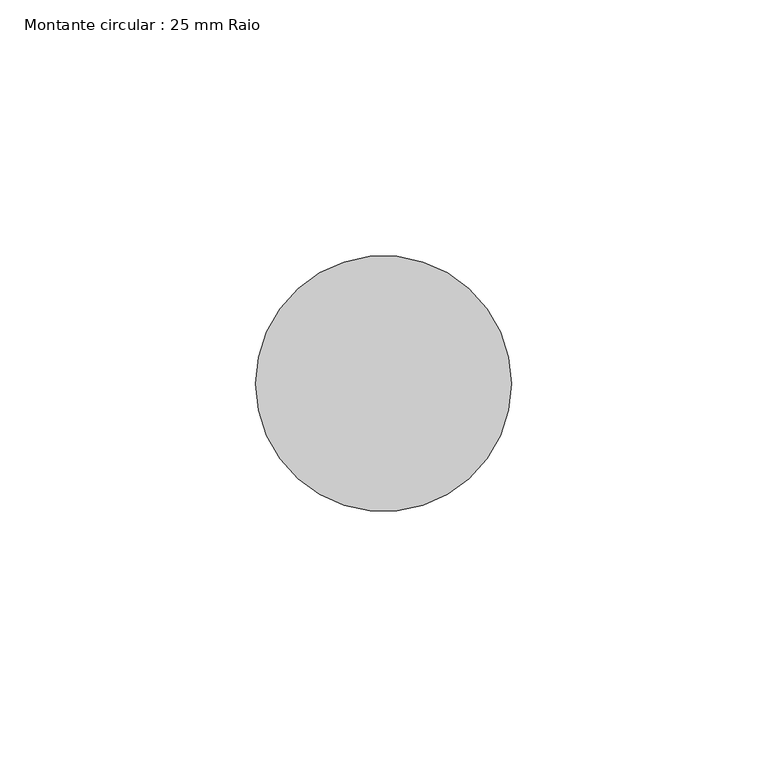
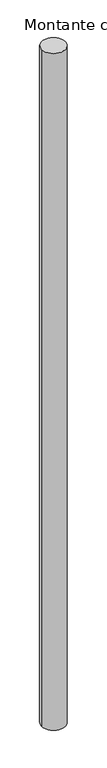
"""IFC4 building model written with IfcOpenShell, lengths in millimetres: member geometry, Montante circular : 25 mm Raio."""

from ifc_helpers import new_model, si_unit, point, frame, frame_2d, origin, place, context, project, spatial, circle_curve, trimmed, segment, composite_curve, outline, extrude, source, transform, mapped, element, save


def montante_circular_25_mm_raio_ce826986(model_context):
    return source(origin(), model_context, "Body", "SweptSolid", [
        extrude(outline(composite_curve([segment(trimmed(circle_curve(frame_2d((-25.0, 0.0)), 25.0), [point((0.0, 0.0))], [point((-50.0, 0.0))], False, "CARTESIAN"), True, "CONTINUOUS"), segment(trimmed(circle_curve(frame_2d((-25.0, 0.0)), 25.0), [point((-50.0, 0.0))], [point((0.0, 0.0))], False, "CARTESIAN"), True, "CONTINUOUS")], self_intersect=False)), frame((0.0, 0.0, -1500.0), z_axis=(0.0, 0.0, 1.0), x_axis=(1.0, 0.0, 0.0)), (0.0, 0.0, 1.0), 1500.0),
    ])


if __name__ == "__main__":
    model = new_model("IFC4")
    model_context = context("Model", 3, world=origin())
    ifc_project = project(units=[si_unit("LENGTHUNIT", "METRE", prefix="MILLI")], contexts=[model_context])
    site = spatial("IfcSite", under=ifc_project)
    building = spatial("IfcBuilding", under=site)
    placement = place(None, origin())
    montante_circular_25_mm_raio_shape = montante_circular_25_mm_raio_ce826986(model_context)
    element("IfcMember", 1, ObjectType="Montante circular : 25 mm Raio", at=placement, inside=building, context=model_context, shape_type="MappedRepresentation", body=[
        mapped(montante_circular_25_mm_raio_shape, transform((0.0, 0.0, 0.0), x_axis=(1.0, 0.0, 0.0), y_axis=(0.0, 1.0, 0.0), z_axis=(0.0, 0.0, 1.0))),
    ])
    save(model, "model.ifc")

# Revit data of these elements
# Type "Montante circular : 25 mm Raio"
#   built-in parameter 1007350 = 0.082021 (stored number, unit not read)
# Element 1 (IfcMember, "Montante circular : 25 mm Raio")
#   Materials on its faces: "Alumín."
# Materials
#   "Alumín.": class "Metal", colour RGB 247 247 247, transparency 0, Description = "Alumín. 6061", Cost = 0
